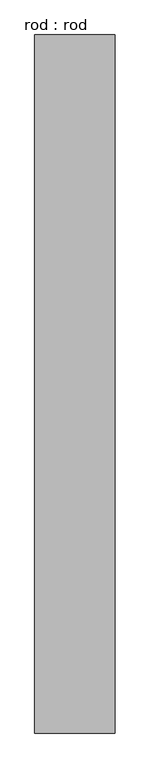
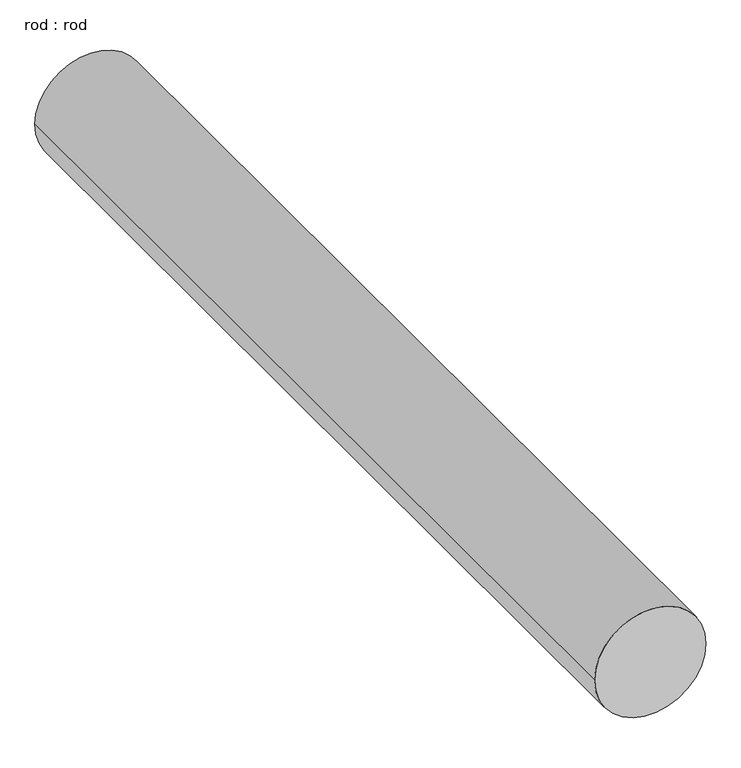
"""IFC4 building model written with IfcOpenShell, lengths in millimetres: proxy geometry, rod : rod."""

from ifc_helpers import new_model, si_unit, point, frame, frame_2d, origin, place, context, project, spatial, circle_curve, trimmed, segment, composite_curve, outline, extrude, source, transform, mapped, element, save


def rod_rod_9ee34040(model_context):
    return source(origin(), model_context, "Body", "SweptSolid", [
        extrude(outline(composite_curve([segment(trimmed(circle_curve(frame_2d((0.0108462, 0.0)), 200.0), [point((0.0108462, 200.0))], [point((0.0108462, -200.0))], False, "CARTESIAN"), True, "CONTINUOUS"), segment(trimmed(circle_curve(frame_2d((0.0108462, 0.0)), 200.0), [point((0.0108462, -200.0))], [point((0.0108462, 200.0))], False, "CARTESIAN"), True, "CONTINUOUS")], self_intersect=False)), frame((0.0, 2351.6571868, 0.0), z_axis=(0.0, 1.0, 0.0), x_axis=(0.0, 0.0, 1.0)), (0.0, 0.0, 1.0), 3482.1428571),
    ])


if __name__ == "__main__":
    model = new_model("IFC4")
    model_context = context("Model", 3, world=origin())
    ifc_project = project(units=[si_unit("LENGTHUNIT", "METRE", prefix="MILLI")], contexts=[model_context])
    site = spatial("IfcSite", under=ifc_project)
    building = spatial("IfcBuilding", under=site)
    placement = place(None, origin())
    rod_rod_shape = rod_rod_9ee34040(model_context)
    element("IfcBuildingElementProxy", 1, Name="rod : rod", ObjectType="rod : rod", at=placement, inside=building, context=model_context, shape_type="MappedRepresentation", body=[
        mapped(rod_rod_shape, transform((0.0, 0.0, 0.0), x_axis=(1.0, 0.0, 0.0), y_axis=(0.0, 1.0, 0.0), z_axis=(0.0, 0.0, 1.0))),
    ])
    save(model, "model.ifc")

# Revit data of these elements
# Type "rod : rod"
#   Default Elevation = 0
